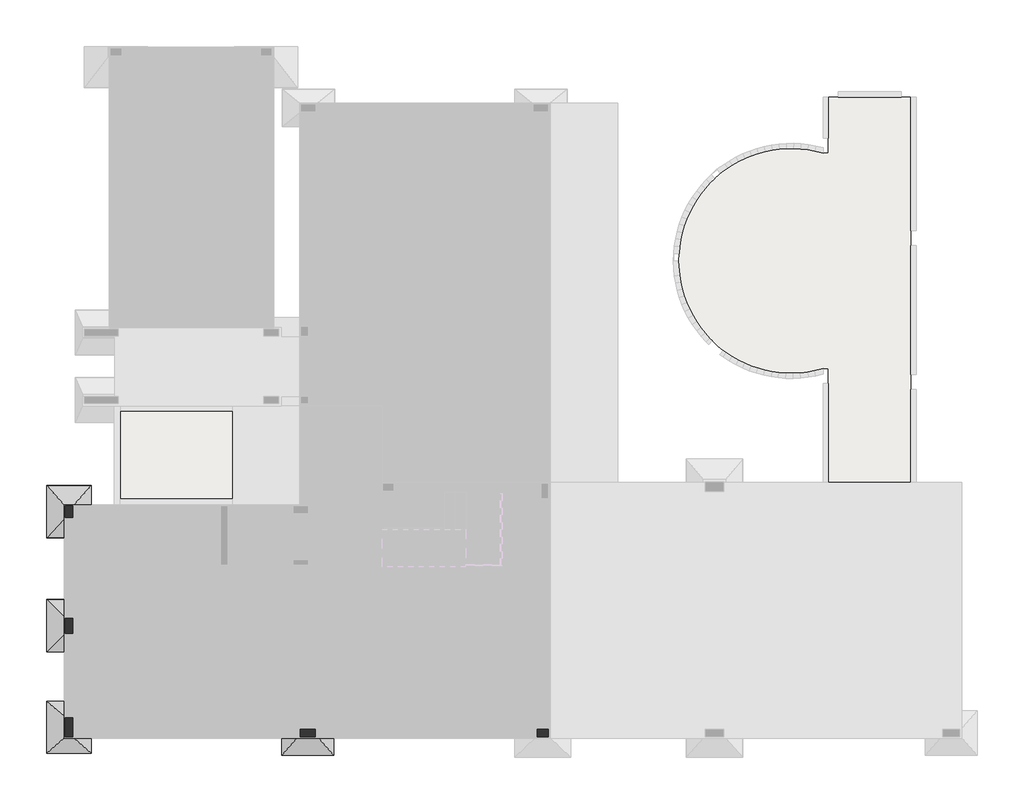
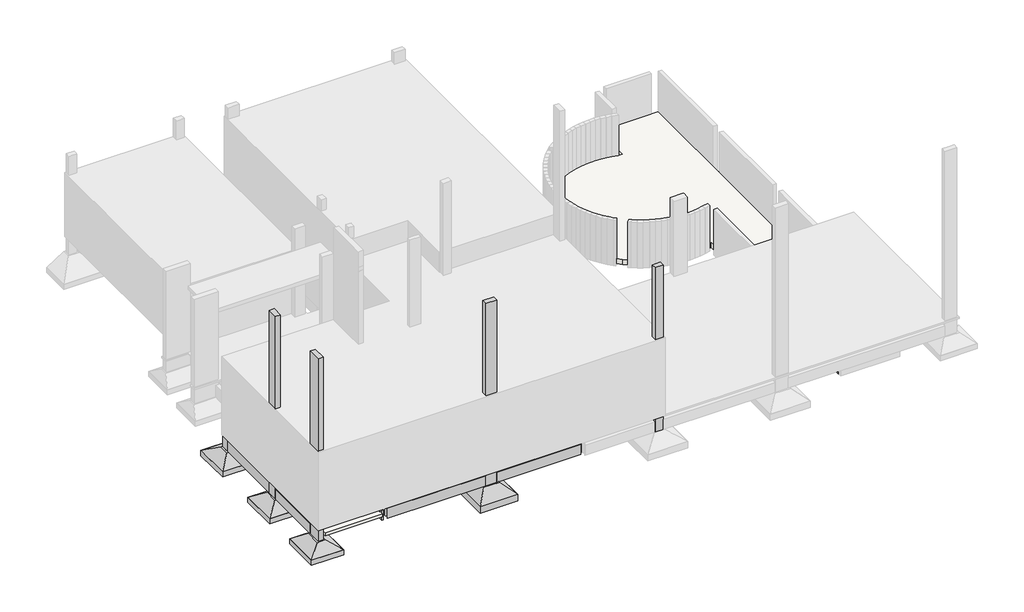
# One storey, part 1 of 4: 11 beams, 5 columns, 4 fasteners, 3 slabs.
# Revit data of these elements (continued)
# Type "TQS - Viga retangular : 14.0 x 40.0"
#   Length [instance default] = 1.524 m
#   b = 0.14 m
#   h = 0.40 m
#   Structural Material [instance default] = none
#   Assembly Code = ""
# Type "TQS - Viga retangular : 19.0 x 40.0"
#   Length [instance default] = 1.524 m
#   b = 0.19 m
#   h = 0.40 m
#   Structural Material [instance default] = none
#   Assembly Code = ""
# Type "TQS - Viga retangular : 19.0 x 55.0"
#   Length [instance default] = 1.524 m
#   b = 0.19 m
#   h = 0.55 m
#   Structural Material [instance default] = none
#   Assembly Code = ""
# Type "TQS - Pilar retangular : 19.0 x 30.0"
#   b = 0.19 m
#   h = 0.30 m
#   Structural Material [instance default] = Concrete - Cast-in-Place Concrete
# Type "TQS - Pilar retangular : 19.0 x 40.0"
#   b = 0.19 m
#   h = 0.40 m
#   Structural Material [instance default] = Concrete - Cast-in-Place Concrete
# Type "TQS - Pilar retangular : 19.0 x 50.0"
#   b = 0.19 m
#   h = 0.50 m
#   Structural Material [instance default] = Concrete - Cast-in-Place Concrete
# Type "TQS - Sapata : S15"
#   TY = 0.40 m
#   TX = 0.29 m
#   HS = 0.50 m
#   H0 = 0.20 m
#   EXCYABS = 0.70 m
#   EXCY = 0.00 m
#   EXCXABS = 0.60 m
#   EXCX = 0.00 m
#   DIMY = 1.40 m
#   DIMX = 1.20 m
#   Material estrutural = Concreto - Concreto concretado no local
#   Width = 0
#   Length = 0
# Type "TQS - Sapata : S19"
#   TY = 0.50 m
#   TX = 0.29 m
#   HS = 0.50 m
#   H0 = 0.20 m
#   EXCYABS = 0.70 m
#   EXCY = 0.00 m
#   EXCXABS = 0.60 m
#   EXCX = 0.00 m
#   DIMY = 1.40 m
#   DIMX = 1.20 m
#   Material estrutural = Concreto - Concreto concretado no local
#   Width = 0
#   Length = 0
# Type "TQS - Sapata : S20"
#   TY = 0.60 m
#   TX = 0.29 m
#   HS = 0.50 m
#   H0 = 0.20 m
#   EXCYABS = 0.70 m
#   EXCY = 0.00 m
#   EXCXABS = 0.60 m
#   EXCX = 0.00 m
#   DIMY = 1.40 m
#   DIMX = 1.20 m
#   Material estrutural = Concreto - Concreto concretado no local
#   Width = 0
#   Length = 0
# Type "TQS - Sapata : S21"
#   TY = 0.60 m
#   TX = 0.29 m
#   HS = 0.60 m
#   H0 = 0.25 m
#   EXCYABS = 0.70 m
#   EXCY = 0.00 m
#   EXCXABS = 0.60 m
#   EXCX = 0.00 m
#   DIMY = 1.40 m
#   DIMX = 1.20 m
#   Material estrutural = Concreto - Concreto concretado no local
#   Width = 0
#   Length = 0
# Type "TQS h=12"
#   Function = 0
#   Layers, outside or top first: 0.12 m ".MATERIAL GENÉRICO LAJE E PISO" (function 1)
# Type "TQS h=20"
#   Function = 0
#   Layers, outside or top first: 0.20 m ".MATERIAL GENÉRICO LAJE E PISO" (function 1)
# Element 1 (IfcBeam, "TQS - Viga retangular : 14.0 x 40.0")
#   Uso = "ESTRUTURA"
#   Titulo = "V22"
#   Chave = "-203"
#   Tipo Elemento = "Viga"
#   SHA1 = "0EE0F179185C4FE731D9B7F49CC743500D79D063"
#   Revisão = ""
#   Tipo de carga = ""
#   Divisor de flexao = ""
#   Secao = ""
#   Configuracao = ""
#   Angulo (graus) = ""
#   Detalhamento = ""
#   Casos de vento manual = ""
#   Tipo = ""
#   Alcas = ""
#   Furos = ""
#   Pino = ""
#   Distribuicao = ""
#   Solidarizado = ""
#   Solidarizar na montagem = ""
#   Unir com o próximo = ""
#   Grupo pre moldado = ""
#   Verificado = ""
#   Concreto C = ""
#   Taxa de armadura (kgf/m³) = 0
#   Carga (tf/m²) = 0
#   Carga (tf/m) = 0
#   Carga (tf) = 0
#   Altura = 0.40 m
#   Rebaixo = 0.07 m
#   Largura = 0.14 m
#   Distancia a face = 0.00 m
#   Distancia ao eixo = 0.00 m
#   Altura gerber esquerda = 0.00 m
#   Largura gerber esquerda = 0.00 m
#   Altura gerber direita = 0.00 m
#   Largura gerber direita = 0.00 m
#   Resultado de Ensaios fck (MPa) = 0
#   Unique TQS ID = -203
#   Principal = yes
#   Structural Material = none
#   Phase Created = CC_AP/ESTR
# Element 2 (IfcBeam, "TQS - Viga retangular : 14.0 x 40.0")
#   Uso = "ESTRUTURA"
#   Titulo = "V9"
#   Chave = "-204"
#   Tipo Elemento = "Viga"
#   SHA1 = "AA57A5F4D00ABE88C47FF187D940E0A6D8A99B36"
#   Revisão = ""
#   Tipo de carga = ""
#   Divisor de flexao = ""
#   Secao = ""
#   Configuracao = ""
#   Angulo (graus) = ""
#   Detalhamento = ""
#   Casos de vento manual = ""
#   Tipo = ""
#   Alcas = ""
#   Furos = ""
#   Pino = ""
#   Distribuicao = ""
#   Solidarizado = ""
#   Solidarizar na montagem = ""
#   Unir com o próximo = ""
#   Grupo pre moldado = ""
#   Verificado = ""
#   Concreto C = ""
#   Taxa de armadura (kgf/m³) = 0
#   Carga (tf/m²) = 0
#   Carga (tf/m) = 0
#   Carga (tf) = 0
#   Altura = 0.40 m
#   Rebaixo = 0.07 m
#   Largura = 0.14 m
#   Distancia a face = 0.00 m
#   Distancia ao eixo = 0.00 m
#   Altura gerber esquerda = 0.00 m
#   Largura gerber esquerda = 0.00 m
#   Altura gerber direita = 0.00 m
#   Largura gerber direita = 0.00 m
#   Resultado de Ensaios fck (MPa) = 0
#   Unique TQS ID = -204
#   Principal = yes
#   Structural Material = none
#   Phase Created = CC_AP/ESTR
# Element 3 (IfcBeam, "TQS - Viga retangular : 14.0 x 40.0")
#   Uso = "ESTRUTURA"
#   Titulo = "V9"
#   Chave = "-205"
#   Tipo Elemento = "Viga"
#   SHA1 = "E87C8EEF9F202EE39708C04CA286767B11167BA7"
#   Revisão = ""
#   Tipo de carga = ""
#   Divisor de flexao = ""
#   Secao = ""
#   Configuracao = ""
#   Angulo (graus) = ""
#   Detalhamento = ""
#   Casos de vento manual = ""
#   Tipo = ""
#   Alcas = ""
#   Furos = ""
#   Pino = ""
#   Distribuicao = ""
#   Solidarizado = ""
#   Solidarizar na montagem = ""
#   Unir com o próximo = ""
#   Grupo pre moldado = ""
#   Verificado = ""
#   Concreto C = ""
#   Taxa de armadura (kgf/m³) = 0
#   Carga (tf/m²) = 0
#   Carga (tf/m) = 0
#   Carga (tf) = 0
#   Altura = 0.40 m
#   Rebaixo = 0.07 m
#   Largura = 0.14 m
#   Distancia a face = 0.00 m
#   Distancia ao eixo = 0.00 m
#   Altura gerber esquerda = 0.00 m
#   Largura gerber esquerda = 0.00 m
#   Altura gerber direita = 0.00 m
#   Largura gerber direita = 0.00 m
#   Resultado de Ensaios fck (MPa) = 0
#   Unique TQS ID = -205
#   Principal = yes
#   Structural Material = none
#   Phase Created = CC_AP/ESTR
# Element 4 (IfcBeam, "TQS - Viga retangular : 14.0 x 40.0")
#   Uso = "ESTRUTURA"
#   Titulo = "V18"
#   Chave = "-208"
#   Tipo Elemento = "Viga"
#   SHA1 = "7D362067162B3A08BECFB8E1D38DC108435A0D97"
#   Revisão = ""
#   Tipo de carga = ""
#   Divisor de flexao = ""
#   Secao = ""
#   Configuracao = ""
#   Angulo (graus) = ""
#   Detalhamento = ""
#   Casos de vento manual = ""
#   Tipo = ""
#   Alcas = ""
#   Furos = ""
#   Pino = ""
#   Distribuicao = ""
#   Solidarizado = ""
#   Solidarizar na montagem = ""
#   Unir com o próximo = ""
#   Grupo pre moldado = ""
#   Verificado = ""
#   Concreto C = ""
#   Taxa de armadura (kgf/m³) = 0
#   Carga (tf/m²) = 0
#   Carga (tf/m) = 0
#   Carga (tf) = 0
#   Altura = 0.40 m
#   Rebaixo = 0.07 m
#   Largura = 0.14 m
#   Distancia a face = 0.00 m
#   Distancia ao eixo = 0.00 m
#   Altura gerber esquerda = 0.00 m
#   Largura gerber esquerda = 0.00 m
#   Altura gerber direita = 0.00 m
#   Largura gerber direita = 0.00 m
#   Resultado de Ensaios fck (MPa) = 0
#   Unique TQS ID = -208
#   Principal = yes
#   Structural Material = none
#   Phase Created = CC_AP/ESTR
# Element 5 (IfcBeam, "TQS - Viga retangular : 14.0 x 40.0")
#   Uso = "ESTRUTURA"
#   Titulo = "V11"
#   Chave = "-212"
#   Tipo Elemento = "Viga"
#   SHA1 = "085A6152135AC5E0DDDC9306F8DBF004F37A3D7F"
#   Revisão = ""
#   Tipo de carga = ""
#   Divisor de flexao = ""
#   Secao = ""
#   Configuracao = ""
#   Angulo (graus) = ""
#   Detalhamento = ""
#   Casos de vento manual = ""
#   Tipo = ""
#   Alcas = ""
#   Furos = ""
#   Pino = ""
#   Distribuicao = ""
#   Solidarizado = ""
#   Solidarizar na montagem = ""
#   Unir com o próximo = ""
#   Grupo pre moldado = ""
#   Verificado = ""
#   Concreto C = ""
#   Taxa de armadura (kgf/m³) = 0
#   Carga (tf/m²) = 0
#   Carga (tf/m) = 0
#   Carga (tf) = 0
#   Altura = 0.40 m
#   Rebaixo = 0.07 m
#   Largura = 0.14 m
#   Distancia a face = 0.00 m
#   Distancia ao eixo = 0.00 m
#   Altura gerber esquerda = 0.00 m
#   Largura gerber esquerda = 0.00 m
#   Altura gerber direita = 0.00 m
#   Largura gerber direita = 0.00 m
#   Resultado de Ensaios fck (MPa) = 0
#   Unique TQS ID = -212
#   Principal = yes
#   Structural Material = none
#   Phase Created = CC_AP/ESTR
# Element 6 (IfcBeam, "TQS - Viga retangular : 14.0 x 40.0")
#   Uso = "ESTRUTURA"
#   Titulo = "V25"
#   Chave = "-214"
#   Tipo Elemento = "Viga"
#   SHA1 = "AA587B3825EEEC75667AA8C6AA5AB994AEC66271"
#   Revisão = ""
#   Tipo de carga = ""
#   Divisor de flexao = ""
#   Secao = ""
#   Configuracao = ""
#   Angulo (graus) = ""
#   Detalhamento = ""
#   Casos de vento manual = ""
#   Tipo = ""
#   Alcas = ""
#   Furos = ""
#   Pino = ""
#   Distribuicao = ""
#   Solidarizado = ""
#   Solidarizar na montagem = ""
#   Unir com o próximo = ""
#   Grupo pre moldado = ""
#   Verificado = ""
#   Concreto C = ""
#   Taxa de armadura (kgf/m³) = 0
#   Carga (tf/m²) = 0
#   Carga (tf/m) = 0
#   Carga (tf) = 0
#   Altura = 0.40 m
#   Rebaixo = 0.16 m
#   Largura = 0.14 m
#   Distancia a face = 0.00 m
#   Distancia ao eixo = 0.00 m
#   Altura gerber esquerda = 0.00 m
#   Largura gerber esquerda = 0.00 m
#   Altura gerber direita = 0.00 m
#   Largura gerber direita = 0.00 m
#   Resultado de Ensaios fck (MPa) = 0
#   Unique TQS ID = -214
#   Principal = yes
#   Structural Material = none
#   Phase Created = CC_AP/ESTR
# Element 7 (IfcBeam, "TQS - Viga retangular : 14.0 x 40.0")
#   Uso = "ESTRUTURA"
#   Titulo = "V12"
#   Chave = "-453"
#   Tipo Elemento = "Viga"
#   SHA1 = "D9CD6F477F2EF098F4AC3262D940A040C72B7E2B"
#   Revisão = ""
#   Tipo de carga = ""
#   Divisor de flexao = ""
#   Secao = ""
#   Configuracao = ""
#   Angulo (graus) = ""
#   Detalhamento = ""
#   Casos de vento manual = ""
#   Tipo = ""
#   Alcas = ""
#   Furos = ""
#   Pino = ""
#   Distribuicao = ""
#   Solidarizado = ""
#   Solidarizar na montagem = ""
#   Unir com o próximo = ""
#   Grupo pre moldado = ""
#   Verificado = ""
#   Concreto C = ""
#   Taxa de armadura (kgf/m³) = 0
#   Carga (tf/m²) = 0
#   Carga (tf/m) = 0
#   Carga (tf) = 0
#   Altura = 0.40 m
#   Rebaixo = 0.16 m
#   Largura = 0.14 m
#   Distancia a face = 0.00 m
#   Distancia ao eixo = 0.00 m
#   Altura gerber esquerda = 0.00 m
#   Largura gerber esquerda = 0.00 m
#   Altura gerber direita = 0.00 m
#   Largura gerber direita = 0.00 m
#   Resultado de Ensaios fck (MPa) = 0
#   Unique TQS ID = -453
#   Principal = yes
#   Structural Material = none
#   Phase Created = CC_AP/ESTR
# Element 8 (IfcBeam, "TQS - Viga retangular : 14.0 x 40.0")
#   Uso = "ESTRUTURA"
#   Titulo = "V13"
#   Chave = "-681"
#   Tipo Elemento = "Viga"
#   SHA1 = "E52B93A2F47D403CA690CD63769ABDF0E8B6050A"
#   Revisão = ""
#   Tipo de carga = ""
#   Divisor de flexao = ""
#   Secao = ""
#   Configuracao = ""
#   Angulo (graus) = ""
#   Detalhamento = ""
#   Casos de vento manual = ""
#   Tipo = ""
#   Alcas = ""
#   Furos = ""
#   Pino = ""
#   Distribuicao = ""
#   Solidarizado = ""
#   Solidarizar na montagem = ""
#   Unir com o próximo = ""
#   Grupo pre moldado = ""
#   Verificado = ""
#   Concreto C = ""
#   Taxa de armadura (kgf/m³) = 0
#   Carga (tf/m²) = 0
#   Carga (tf/m) = 0
#   Carga (tf) = 0
#   Altura = 0.40 m
#   Rebaixo = 0.07 m
#   Largura = 0.14 m
#   Distancia a face = 0.00 m
#   Distancia ao eixo = 0.00 m
#   Altura gerber esquerda = 0.00 m
#   Largura gerber esquerda = 0.00 m
#   Altura gerber direita = 0.00 m
#   Largura gerber direita = 0.00 m
#   Resultado de Ensaios fck (MPa) = 0
#   Unique TQS ID = -681
#   Principal = yes
#   Structural Material = none
#   Phase Created = CC_AP/ESTR
# Element 9 (IfcBeam, "TQS - Viga retangular : 19.0 x 40.0")
#   Uso = "ESTRUTURA"
#   Titulo = "V16"
#   Chave = "-181"
#   Tipo Elemento = "Viga"
#   SHA1 = "AC6EE286E954C664F8248081444A5D98129228D8"
#   Revisão = ""
#   Tipo de carga = ""
#   Divisor de flexao = ""
#   Secao = ""
#   Configuracao = ""
#   Angulo (graus) = ""
#   Detalhamento = ""
#   Casos de vento manual = ""
#   Tipo = ""
#   Alcas = ""
#   Furos = ""
#   Pino = ""
#   Distribuicao = ""
#   Solidarizado = ""
#   Solidarizar na montagem = ""
#   Unir com o próximo = ""
#   Grupo pre moldado = ""
#   Verificado = ""
#   Concreto C = ""
#   Taxa de armadura (kgf/m³) = 0
#   Carga (tf/m²) = 0
#   Carga (tf/m) = 0
#   Carga (tf) = 0
#   Altura = 0.40 m
#   Rebaixo = 0.07 m
#   Largura = 0.19 m
#   Distancia a face = 0.00 m
#   Distancia ao eixo = 0.00 m
#   Altura gerber esquerda = 0.00 m
#   Largura gerber esquerda = 0.00 m
#   Altura gerber direita = 0.00 m
#   Largura gerber direita = 0.00 m
#   Resultado de Ensaios fck (MPa) = 0
#   Unique TQS ID = -181
#   Principal = yes
#   Structural Material = none
#   Phase Created = CC_AP/ESTR
# Element 10 (IfcBeam, "TQS - Viga retangular : 19.0 x 40.0")
#   Uso = "ESTRUTURA"
#   Titulo = "V14"
#   Chave = "-188"
#   Tipo Elemento = "Viga"
#   SHA1 = "7A53358B50FB0481EBEA1D15A12D2A0FCC9FC715"
#   Revisão = ""
#   Tipo de carga = ""
#   Divisor de flexao = ""
#   Secao = ""
#   Configuracao = ""
#   Angulo (graus) = ""
#   Detalhamento = ""
#   Casos de vento manual = ""
#   Tipo = ""
#   Alcas = ""
#   Furos = ""
#   Pino = ""
#   Distribuicao = ""
#   Solidarizado = ""
#   Solidarizar na montagem = ""
#   Unir com o próximo = ""
#   Grupo pre moldado = ""
#   Verificado = ""
#   Concreto C = ""
#   Taxa de armadura (kgf/m³) = 0
#   Carga (tf/m²) = 0
#   Carga (tf/m) = 0
#   Carga (tf) = 0
#   Altura = 0.40 m
#   Rebaixo = 0.07 m
#   Largura = 0.19 m
#   Distancia a face = 0.00 m
#   Distancia ao eixo = 0.00 m
#   Altura gerber esquerda = 0.00 m
#   Largura gerber esquerda = 0.00 m
#   Altura gerber direita = 0.00 m
#   Largura gerber direita = 0.00 m
#   Resultado de Ensaios fck (MPa) = 0
#   Unique TQS ID = -188
#   Principal = yes
#   Structural Material = none
#   Phase Created = CC_AP/ESTR
# Element 11 (IfcBeam, "TQS - Viga retangular : 19.0 x 55.0")
#   Uso = "ESTRUTURA"
#   Titulo = "V7"
#   Chave = "-184"
#   Tipo Elemento = "Viga"
#   SHA1 = "E9EC7280BBA3FFEC13DD100B26C6CC66CFF47B76"
#   Revisão = ""
#   Tipo de carga = ""
#   Divisor de flexao = ""
#   Secao = ""
#   Configuracao = ""
#   Angulo (graus) = ""
#   Detalhamento = ""
#   Casos de vento manual = ""
#   Tipo = ""
#   Alcas = ""
#   Furos = ""
#   Pino = ""
#   Distribuicao = ""
#   Solidarizado = ""
#   Solidarizar na montagem = ""
#   Unir com o próximo = ""
#   Grupo pre moldado = ""
#   Verificado = ""
#   Concreto C = ""
#   Taxa de armadura (kgf/m³) = 0
#   Carga (tf/m²) = 0
#   Carga (tf/m) = 0
#   Carga (tf) = 0
#   Altura = 0.55 m
#   Rebaixo = 0.07 m
#   Largura = 0.19 m
#   Distancia a face = 0.00 m
#   Distancia ao eixo = 0.00 m
#   Altura gerber esquerda = 0.00 m
#   Largura gerber esquerda = 0.00 m
#   Altura gerber direita = 0.00 m
#   Largura gerber direita = 0.00 m
#   Resultado de Ensaios fck (MPa) = 0
#   Unique TQS ID = -184
#   Principal = yes
#   Structural Material = none
#   Phase Created = CC_AP/ESTR
# Element 12 (IfcColumn, "TQS - Pilar retangular : 19.0 x 30.0")
#   Uso = "ESTRUTURA"
#   Titulo = "P22"
#   Chave = "P22//0"
#   Tipo Elemento = "Pilar"
#   SHA1 = "74B32C051183367140A14ED156F148A997E93745"
#   Revisão = ""
#   Tipo de carga = ""
#   Divisor de flexao = ""
#   Secao = "R 19/30 90°"
#   Configuracao = ""
#   Angulo (graus) = ""
#   Detalhamento = ""
#   Casos de vento manual = ""
#   Tipo = ""
#   Alcas = ""
#   Furos = ""
#   Pino = ""
#   Distribuicao = ""
#   Solidarizado = ""
#   Solidarizar na montagem = ""
#   Unir com o próximo = ""
#   Grupo pre moldado = ""
#   Verificado = ""
#   Concreto C = ""
#   Taxa de armadura (kgf/m³) = 0
#   Carga (tf/m²) = 0
#   Carga (tf/m) = 0
#   Carga (tf) = 0
#   Altura = 8.25 m
#   Rebaixo = 0.00 m
#   Altura da fundacao = 0.00 m
#   Largura = 0.00 m
#   Distancia a face = 0.00 m
#   Distancia ao eixo = 0.00 m
#   Resultado de Ensaios fck (MPa) = 0
#   Unique TQS ID = -52
#   Principal = yes
#   Nasce = yes
#   Morre = yes
#   Cabeca de Pilar = no
#   Structural Material = Concrete - Cast-in-Place Concrete
#   Phase Created = CC_AP/ESTR
#   Materials on its faces: "Concrete - Cast-in-Place Concrete"
# Element 13 (IfcColumn, "TQS - Pilar retangular : 19.0 x 30.0")
#   Uso = "ESTRUTURA"
#   Titulo = "P15"
#   Chave = "P15//0"
#   Tipo Elemento = "Pilar"
#   SHA1 = "E1EF40F284DB4178944633D19F269044313D4902"
#   Revisão = ""
#   Tipo de carga = ""
#   Divisor de flexao = ""
#   Secao = "R 19/30"
#   Configuracao = ""
#   Angulo (graus) = ""
#   Detalhamento = ""
#   Casos de vento manual = ""
#   Tipo = ""
#   Alcas = ""
#   Furos = ""
#   Pino = ""
#   Distribuicao = ""
#   Solidarizado = ""
#   Solidarizar na montagem = ""
#   Unir com o próximo = ""
#   Grupo pre moldado = ""
#   Verificado = ""
#   Concreto C = ""
#   Taxa de armadura (kgf/m³) = 0
#   Carga (tf/m²) = 0
#   Carga (tf/m) = 0
#   Carga (tf) = 0
#   Altura = 3.10 m
#   Rebaixo = 0.00 m
#   Altura da fundacao = 0.00 m
#   Largura = 0.00 m
#   Distancia a face = 0.00 m
#   Distancia ao eixo = 0.00 m
#   Resultado de Ensaios fck (MPa) = 0
#   Unique TQS ID = -165
#   Principal = yes
#   Nasce = yes
#   Morre = yes
#   Cabeca de Pilar = no
#   Structural Material = Concrete - Cast-in-Place Concrete
#   Phase Created = CC_AP/ESTR
#   Materials on its faces: "Concrete - Cast-in-Place Concrete"
# Element 14 (IfcColumn, "TQS - Pilar retangular : 19.0 x 40.0")
#   Uso = "ESTRUTURA"
#   Titulo = "P19"
#   Chave = "P19//0"
#   Tipo Elemento = "Pilar"
#   SHA1 = "093B358AFDBAA251B04AA547A5D91A122216BA95"
#   Revisão = ""
#   Tipo de carga = ""
#   Divisor de flexao = ""
#   Secao = "R 19/40"
#   Configuracao = ""
#   Angulo (graus) = ""
#   Detalhamento = ""
#   Casos de vento manual = ""
#   Tipo = ""
#   Alcas = ""
#   Furos = ""
#   Pino = ""
#   Distribuicao = ""
#   Solidarizado = ""
#   Solidarizar na montagem = ""
#   Unir com o próximo = ""
#   Grupo pre moldado = ""
#   Verificado = ""
#   Concreto C = ""
#   Taxa de armadura (kgf/m³) = 0
#   Carga (tf/m²) = 0
#   Carga (tf/m) = 0
#   Carga (tf) = 0
#   Altura = 6.15 m
#   Rebaixo = 0.00 m
#   Altura da fundacao = 0.00 m
#   Largura = 0.00 m
#   Distancia a face = 0.00 m
#   Distancia ao eixo = 0.00 m
#   Resultado de Ensaios fck (MPa) = 0
#   Unique TQS ID = -55
#   Principal = yes
#   Nasce = yes
#   Morre = yes
#   Cabeca de Pilar = no
#   Structural Material = Concrete - Cast-in-Place Concrete
#   Phase Created = CC_AP/ESTR
#   Materials on its faces: "Concrete - Cast-in-Place Concrete"
# Element 15 (IfcColumn, "TQS - Pilar retangular : 19.0 x 40.0")
#   Uso = "ESTRUTURA"
#   Titulo = "P21"
#   Chave = "P21//0"
#   Tipo Elemento = "Pilar"
#   SHA1 = "7EA026137CEA6DD5128C297612ADEF5773B66F62"
#   Revisão = ""
#   Tipo de carga = ""
#   Divisor de flexao = ""
#   Secao = "R 19/40 270°"
#   Configuracao = ""
#   Angulo (graus) = ""
#   Detalhamento = ""
#   Casos de vento manual = ""
#   Tipo = ""
#   Alcas = ""
#   Furos = ""
#   Pino = ""
#   Distribuicao = ""
#   Solidarizado = ""
#   Solidarizar na montagem = ""
#   Unir com o próximo = ""
#   Grupo pre moldado = ""
#   Verificado = ""
#   Concreto C = ""
#   Taxa de armadura (kgf/m³) = 0
#   Carga (tf/m²) = 0
#   Carga (tf/m) = 0
#   Carga (tf) = 0
#   Altura = 6.15 m
#   Rebaixo = 0.00 m
#   Altura da fundacao = 0.00 m
#   Largura = 0.00 m
#   Distancia a face = 0.00 m
#   Distancia ao eixo = 0.00 m
#   Resultado de Ensaios fck (MPa) = 0
#   Unique TQS ID = -166
#   Principal = yes
#   Nasce = yes
#   Morre = yes
#   Cabeca de Pilar = no
#   Structural Material = Concrete - Cast-in-Place Concrete
#   Phase Created = CC_AP/ESTR
#   Materials on its faces: "Concrete - Cast-in-Place Concrete"
# Element 16 (IfcColumn, "TQS - Pilar retangular : 19.0 x 50.0")
#   Uso = "ESTRUTURA"
#   Titulo = "P20"
#   Chave = "P20//0"
#   Tipo Elemento = "Pilar"
#   SHA1 = "CBA1581784D1834A270D99BD43DC7DB390139A31"
#   Revisão = ""
#   Tipo de carga = ""
#   Divisor de flexao = ""
#   Secao = "R 19/50"
#   Configuracao = ""
#   Angulo (graus) = ""
#   Detalhamento = ""
#   Casos de vento manual = ""
#   Tipo = ""
#   Alcas = ""
#   Furos = ""
#   Pino = ""
#   Distribuicao = ""
#   Solidarizado = ""
#   Solidarizar na montagem = ""
#   Unir com o próximo = ""
#   Grupo pre moldado = ""
#   Verificado = ""
#   Concreto C = ""
#   Taxa de armadura (kgf/m³) = 0
#   Carga (tf/m²) = 0
#   Carga (tf/m) = 0
#   Carga (tf) = 0
#   Altura = 6.15 m
#   Rebaixo = 0.00 m
#   Altura da fundacao = 0.00 m
#   Largura = 0.00 m
#   Distancia a face = 0.00 m
#   Distancia ao eixo = 0.00 m
#   Resultado de Ensaios fck (MPa) = 0
#   Unique TQS ID = -54
#   Principal = yes
#   Nasce = yes
#   Morre = yes
#   Cabeca de Pilar = no
#   Structural Material = Concrete - Cast-in-Place Concrete
#   Phase Created = CC_AP/ESTR
#   Materials on its faces: "Concrete - Cast-in-Place Concrete"
# Element 17 (IfcFastener, "TQS - Sapata : S15")
#   Uso = "ESTRUTURA"
#   Titulo = "S15"
#   Chave = "-1472"
#   Tipo Elemento = "Fundação"
#   SHA1 = "D4CAB0671F7DE7F29C2B2445B1EEE28D1894D6FF"
#   Revisão = ""
#   Tipo de carga = ""
#   Divisor de flexao = ""
#   Secao = ""
#   Configuracao = ""
#   Angulo (graus) = ""
#   Detalhamento = ""
#   Casos de vento manual = ""
#   Tipo = "Sapata"
#   Dimensoes = "120.0,140.0"
#   Estacas = ""
#   Calice = ""
#   Rugosidade = ""
#   Alcas = ""
#   Furos = ""
#   Pino = ""
#   Distribuicao = ""
#   Solidarizado = ""
#   Solidarizar na montagem = ""
#   Unir com o próximo = ""
#   Grupo pre moldado = ""
#   Verificado = ""
#   Concreto C = ""
#   Taxa de armadura (kgf/m³) = 0
#   Carga (tf/m²) = 0
#   Carga (tf/m) = 0
#   Carga (tf) = 0
#   Altura = 0.00 m
#   Rebaixo = 0.00 m
#   Pilar ficticio = 0.00 m
#   Topo = 0.03 m
#   Altura total = 0.50 m
#   Rodape = 0.00 m
#   Diametro = 0.00 m
#   Altura dentro do bloco = 0.00 m
#   Entre eixos = 0.00 m
#   Paredes = 0.00 m
#   Caimento = 0.00 m
#   Largura = 0.00 m
#   Distancia a face = 0.00 m
#   Distancia ao eixo = 0.00 m
#   Resultado de Ensaios fck (MPa) = 0
#   Unique TQS ID = -1472
#   Principal = yes
#   Phase Created = CC_AP/ESTR
#   Materials on its faces: "Concreto - Concreto concretado no local"
# Element 18 (IfcFastener, "TQS - Sapata : S19")
#   Uso = "ESTRUTURA"
#   Titulo = "S19"
#   Chave = "-1464"
#   Tipo Elemento = "Fundação"
#   SHA1 = "696692FDA33825790091079D26A0FC1744923CA0"
#   Revisão = ""
#   Tipo de carga = ""
#   Divisor de flexao = ""
#   Secao = ""
#   Configuracao = ""
#   Angulo (graus) = ""
#   Detalhamento = ""
#   Casos de vento manual = ""
#   Tipo = "Sapata"
#   Dimensoes = "120.0,140.0"
#   Estacas = ""
#   Calice = ""
#   Rugosidade = ""
#   Alcas = ""
#   Furos = ""
#   Pino = ""
#   Distribuicao = ""
#   Solidarizado = ""
#   Solidarizar na montagem = ""
#   Unir com o próximo = ""
#   Grupo pre moldado = ""
#   Verificado = ""
#   Concreto C = ""
#   Taxa de armadura (kgf/m³) = 0
#   Carga (tf/m²) = 0
#   Carga (tf/m) = 0
#   Carga (tf) = 0
#   Altura = 0.00 m
#   Rebaixo = 0.00 m
#   Pilar ficticio = 0.00 m
#   Topo = 0.03 m
#   Altura total = 0.50 m
#   Rodape = 0.00 m
#   Diametro = 0.00 m
#   Altura dentro do bloco = 0.00 m
#   Entre eixos = 0.00 m
#   Paredes = 0.00 m
#   Caimento = 0.00 m
#   Largura = 0.00 m
#   Distancia a face = 0.00 m
#   Distancia ao eixo = 0.00 m
#   Resultado de Ensaios fck (MPa) = 0
#   Unique TQS ID = -1464
#   Principal = yes
#   Phase Created = CC_AP/ESTR
#   Materials on its faces: "Concreto - Concreto concretado no local"
# Element 19 (IfcFastener, "TQS - Sapata : S20")
#   Uso = "ESTRUTURA"
#   Titulo = "S20"
#   Chave = "-1462"
#   Tipo Elemento = "Fundação"
#   SHA1 = "E8A55F044D5D0FEDAF3A2E52ADD3CCB0BA977F38"
#   Revisão = ""
#   Tipo de carga = ""
#   Divisor de flexao = ""
#   Secao = ""
#   Configuracao = ""
#   Angulo (graus) = ""
#   Detalhamento = ""
#   Casos de vento manual = ""
#   Tipo = "Sapata"
#   Dimensoes = "120.0,140.0"
#   Estacas = ""
#   Calice = ""
#   Rugosidade = ""
#   Alcas = ""
#   Furos = ""
#   Pino = ""
#   Distribuicao = ""
#   Solidarizado = ""
#   Solidarizar na montagem = ""
#   Unir com o próximo = ""
#   Grupo pre moldado = ""
#   Verificado = ""
#   Concreto C = ""
#   Taxa de armadura (kgf/m³) = 0
#   Carga (tf/m²) = 0
#   Carga (tf/m) = 0
#   Carga (tf) = 0
#   Altura = 0.00 m
#   Rebaixo = 0.00 m
#   Pilar ficticio = 0.00 m
#   Topo = 0.03 m
#   Altura total = 0.50 m
#   Rodape = 0.00 m
#   Diametro = 0.00 m
#   Altura dentro do bloco = 0.00 m
#   Entre eixos = 0.00 m
#   Paredes = 0.00 m
#   Caimento = 0.00 m
#   Largura = 0.00 m
#   Distancia a face = 0.00 m
#   Distancia ao eixo = 0.00 m
#   Resultado de Ensaios fck (MPa) = 0
#   Unique TQS ID = -1462
#   Principal = yes
#   Phase Created = CC_AP/ESTR
#   Materials on its faces: "Concreto - Concreto concretado no local"
# Element 20 (IfcFastener, "TQS - Sapata : S21")
#   Uso = "ESTRUTURA"
#   Titulo = "S21"
#   Chave = "-1463"
#   Tipo Elemento = "Fundação"
#   SHA1 = "0C6532C4A6A661814370FBEABFA2346616E70F6C"
#   Revisão = ""
#   Tipo de carga = ""
#   Divisor de flexao = ""
#   Secao = ""
#   Configuracao = ""
#   Angulo (graus) = ""
#   Detalhamento = ""
#   Casos de vento manual = ""
#   Tipo = "Sapata"
#   Dimensoes = "120.0,140.0"
#   Estacas = ""
#   Calice = ""
#   Rugosidade = ""
#   Alcas = ""
#   Furos = ""
#   Pino = ""
#   Distribuicao = ""
#   Solidarizado = ""
#   Solidarizar na montagem = ""
#   Unir com o próximo = ""
#   Grupo pre moldado = ""
#   Verificado = ""
#   Concreto C = ""
#   Taxa de armadura (kgf/m³) = 0
#   Carga (tf/m²) = 0
#   Carga (tf/m) = 0
#   Carga (tf) = 0
#   Altura = 0.00 m
#   Rebaixo = 0.00 m
#   Pilar ficticio = 0.00 m
#   Topo = 0.03 m
#   Altura total = 0.60 m
#   Rodape = 0.00 m
#   Diametro = 0.00 m
#   Altura dentro do bloco = 0.00 m
#   Entre eixos = 0.00 m
#   Paredes = 0.00 m
#   Caimento = 0.00 m
#   Largura = 0.00 m
#   Distancia a face = 0.00 m
#   Distancia ao eixo = 0.00 m
#   Resultado de Ensaios fck (MPa) = 0
#   Unique TQS ID = -1463
#   Principal = yes
#   Phase Created = CC_AP/ESTR
#   Materials on its faces: "Concreto - Concreto concretado no local"
# Element 21 (IfcSlab, "TQS h=12")
#   Uso = "ESTRUTURA"
#   Titulo = "L2"
#   Chave = "-541"
#   Tipo Elemento = "Laje"
#   SHA1 = "9D88A251886EA259D37D7D6526C24190D18449DE"
#   Revisão = ""
#   Tipo de carga = ""
#   Divisor de flexao = ""
#   Fabricante = ""
#   Enchimento = ""
#   Mini painel = ""
#   Blocos por nervura = ""
#   Secao = ""
#   Configuracao = ""
#   Angulo (graus) = "0"
#   Detalhamento = ""
#   Casos de vento manual = ""
#   Tipo = "Maciça"
#   Alcas = ""
#   Furos = ""
#   Pino = ""
#   Distribuicao = ""
#   Solidarizado = ""
#   Solidarizar na montagem = ""
#   Unir com o próximo = ""
#   Grupo pre moldado = ""
#   Verificado = ""
#   Concreto C = ""
#   Height Offset From Level = -0.50 m
#   Taxa de armadura (kgf/m³) = 0
#   Carga (tf/m²) = 0
#   Carga (tf/m) = 0
#   Carga (tf) = 0
#   Altura = 0.12 m
#   Capa = 0.00 m
#   Capa inferior = 0.00 m
#   Altura da nervura = 0.00 m
#   Enchimento (tf/m³) = 0
#   Largura inferior X = 0.00 m
#   Distancia inferior X = 0.00 m
#   Largura inferior Y = 0.00 m
#   Distancia inferior Y = 0.00 m
#   Largura vigota = 0.00 m
#   Altura vigota = 0.00 m
#   Largura perfil = 0.00 m
#   Largura aba = 0.00 m
#   Altura perfil = 0.00 m
#   Nervura secundaria = 0.00 m
#   Desconto nervura secundaria = 0.00 m
#   Rebaixo = -0.50 m
#   Largura = 0.00 m
#   Distancia a face = 0.00 m
#   Distancia ao eixo = 0.00 m
#   Resultado de Ensaios fck (MPa) = 0
#   built-in parameter 1001954 = 1
#   Unique TQS ID = -541
#   Principal = yes
#   Phase Created = CC_AP/ESTR
#   Materials on its faces: ".MATERIAL GENÉRICO LAJE E PISO"
# Element 22 (IfcSlab, "TQS h=12")
#   Uso = "ESTRUTURA"
#   Titulo = "L8"
#   Chave = "-680"
#   Tipo Elemento = "Laje"
#   SHA1 = "9859310AA961365E5B9659041FB058FECACF80B9"
#   Revisão = ""
#   Tipo de carga = ""
#   Divisor de flexao = ""
#   Fabricante = ""
#   Enchimento = ""
#   Mini painel = ""
#   Blocos por nervura = ""
#   Secao = ""
#   Configuracao = ""
#   Angulo (graus) = "0"
#   Detalhamento = ""
#   Casos de vento manual = ""
#   Tipo = "Maciça"
#   Alcas = ""
#   Furos = ""
#   Pino = ""
#   Distribuicao = ""
#   Solidarizado = ""
#   Solidarizar na montagem = ""
#   Unir com o próximo = ""
#   Grupo pre moldado = ""
#   Verificado = ""
#   Concreto C = ""
#   Height Offset From Level = -0.18 m
#   Taxa de armadura (kgf/m³) = 0
#   Carga (tf/m²) = 0
#   Carga (tf/m) = 0
#   Carga (tf) = 0
#   Altura = 0.12 m
#   Capa = 0.00 m
#   Capa inferior = 0.00 m
#   Altura da nervura = 0.00 m
#   Enchimento (tf/m³) = 0
#   Largura inferior X = 0.00 m
#   Distancia inferior X = 0.00 m
#   Largura inferior Y = 0.00 m
#   Distancia inferior Y = 0.00 m
#   Largura vigota = 0.00 m
#   Altura vigota = 0.00 m
#   Largura perfil = 0.00 m
#   Largura aba = 0.00 m
#   Altura perfil = 0.00 m
#   Nervura secundaria = 0.00 m
#   Desconto nervura secundaria = 0.00 m
#   Rebaixo = -0.18 m
#   Largura = 0.00 m
#   Distancia a face = 0.00 m
#   Distancia ao eixo = 0.00 m
#   Resultado de Ensaios fck (MPa) = 0
#   built-in parameter 1001954 = 1
#   Unique TQS ID = -680
#   Principal = yes
#   Phase Created = CC_AP/ESTR
#   Materials on its faces: ".MATERIAL GENÉRICO LAJE E PISO"
# Element 23 (IfcSlab, "TQS h=20")
#   Uso = "ESTRUTURA"
#   Titulo = "L4"
#   Chave = "-843"
#   Tipo Elemento = "Laje"
#   SHA1 = "FB4864774B549ABE2AC3E52C0811E4BD1C9F7941"
#   Revisão = ""
#   Tipo de carga = ""
#   Divisor de flexao = ""
#   Fabricante = ""
#   Enchimento = ""
#   Mini painel = ""
#   Blocos por nervura = ""
#   Secao = ""
#   Configuracao = ""
#   Angulo (graus) = "0"
#   Detalhamento = ""
#   Casos de vento manual = ""
#   Tipo = "Maciça"
#   Alcas = ""
#   Furos = ""
#   Pino = ""
#   Distribuicao = ""
#   Solidarizado = ""
#   Solidarizar na montagem = ""
#   Unir com o próximo = ""
#   Grupo pre moldado = ""
#   Verificado = ""
#   Concreto C = ""
#   Height Offset From Level = -1.75 m
#   Taxa de armadura (kgf/m³) = 0
#   Carga (tf/m²) = 0
#   Carga (tf/m) = 0
#   Carga (tf) = 0
#   Altura = 0.20 m
#   Capa = 0.00 m
#   Capa inferior = 0.00 m
#   Altura da nervura = 0.00 m
#   Enchimento (tf/m³) = 0
#   Largura inferior X = 0.00 m
#   Distancia inferior X = 0.00 m
#   Largura inferior Y = 0.00 m
#   Distancia inferior Y = 0.00 m
#   Largura vigota = 0.00 m
#   Altura vigota = 0.00 m
#   Largura perfil = 0.00 m
#   Largura aba = 0.00 m
#   Altura perfil = 0.00 m
#   Nervura secundaria = 0.00 m
#   Desconto nervura secundaria = 0.00 m
#   Rebaixo = -1.75 m
#   Largura = 0.00 m
#   Distancia a face = 0.00 m
#   Distancia ao eixo = 0.00 m
#   Resultado de Ensaios fck (MPa) = 0
#   built-in parameter 1001954 = 1
#   Unique TQS ID = -843
#   Principal = yes
#   Phase Created = CC_AP/ESTR
#   Materials on its faces: ".MATERIAL GENÉRICO LAJE E PISO"
# Materials
#   "Concrete - Cast-in-Place Concrete": class "Unassigned", colour RGB 192 192 192, transparency 0
#   "Concreto - Concreto concretado no local": class "Concreto", colour RGB 192 192 192, transparency 0
#   ".MATERIAL GENÉRICO LAJE E PISO": class ".CC_PAVIMENTAÇÃO", colour RGB 128 128 128, transparency 0, Description = "Material genérico para representação ND 200.", Cost = 0
